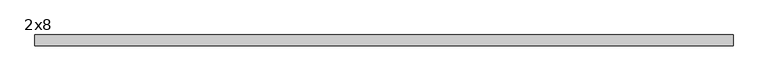
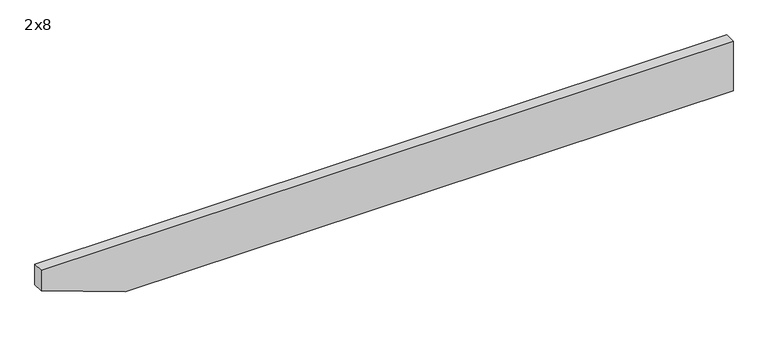
"""IFC4 building model written with IfcOpenShell, lengths in millimetres: beam geometry, Dimension Lumber - Truncated : 2x8."""

from ifc_helpers import new_model, si_unit, frame, origin, place, context, project, spatial, polyline, outline, extrude, source, transform, mapped, element, save


def beam_2x8_64904455(model_context):
    return source(origin(), model_context, "Body", "SweptSolid", [
        extrude(outline(polyline([(-92.075, 1219.2), (92.075, 1219.2), (92.075, -1219.2), (15.875, -1219.2), (-92.075, -922.6098126), (-92.075, 1219.2)])), frame((0.0, -19.05, 0.0), z_axis=(0.0, 1.0, 0.0), x_axis=(0.0, 0.0, 1.0)), (0.0, 0.0, 1.0), 38.1),
    ])


if __name__ == "__main__":
    model = new_model("IFC4")
    model_context = context("Model", 3, world=origin())
    ifc_project = project(units=[si_unit("LENGTHUNIT", "METRE", prefix="MILLI")], contexts=[model_context])
    site = spatial("IfcSite", under=ifc_project)
    building = spatial("IfcBuilding", under=site)
    placement = place(None, origin())
    beam_2x8_shape = beam_2x8_64904455(model_context)
    element("IfcBeam", 1, ObjectType="Dimension Lumber - Truncated : 2x8", at=placement, inside=building, context=model_context, shape_type="MappedRepresentation", body=[
        mapped(beam_2x8_shape, transform((0.0, 0.0, 0.0), x_axis=(1.0, 0.0, 0.0), y_axis=(0.0, 1.0, 0.0), z_axis=(0.0, 0.0, 1.0))),
    ])
    save(model, "model.ifc")

# Revit data of these elements
# Type "Dimension Lumber - Truncated : 2x8"
#   Assembly Code = "B10"
#   Leading Edge Dimension = 0' - 3"
#   Start Angle = 70.00°
#   End Angle = 0.00°
#   A = 0.0755556 SF
#   Length [instance default] = 5' - 0"
#   b = 0' - 1 1/2"
#   d = 0' - 7 1/4"
#   Structural Material = Softwood, Lumber - hortz
# Element 1 (IfcBeam, "Dimension Lumber - Truncated : 2x8")
#   Materials on its faces: "Softwood, Lumber - hortz"
# Materials
#   "Softwood, Lumber - hortz": class "Wood", colour RGB 131 91 56, transparency 0, Description = "Pinus Echinata", Cost = 0
